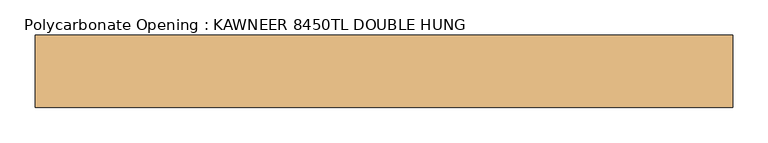
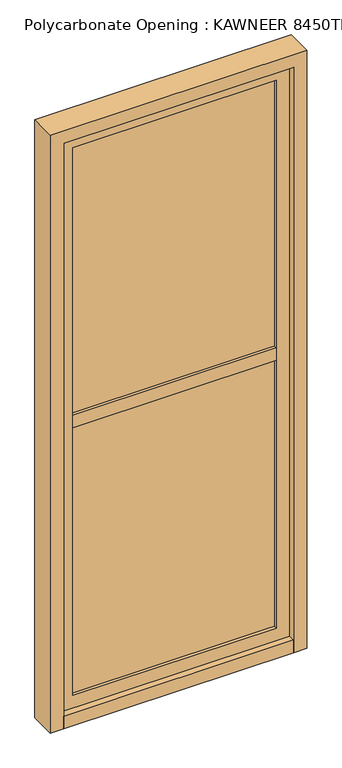
"""IFC4 building model written with IfcOpenShell, lengths in millimetres: door geometry, Polycarbonate Opening : KAWNEER 8450TL DOUBLE HUNG."""

from ifc_helpers import new_model, si_unit, frame, origin, origin_with_axes, place, context, project, spatial, polyline, outline, extrude, source, transform, mapped, element, save


def polycarbonate_opening_kawneer_8450tl_double_hung_a71d8d07(model_context):
    return source(origin(), model_context, "Body", "SweptSolid", [
        extrude(outline(polyline([(440.1908884, 12.7), (440.1908884, -12.7), (-440.1908884, -12.7), (-440.1908884, 12.7), (440.1908884, 12.7)])), frame((0.0, 0.0, 50.8), z_axis=(0.0, 0.0, 1.0), x_axis=(1.0, 0.0, 0.0)), (0.0, 0.0, 1.0), 2318.3403955),
        extrude(outline(polyline([(2369.1403955, -440.1908884), (0.0, -440.1908884), (0.0, 440.1908884), (2369.1403955, 440.1908884), (2369.1403955, -440.1908884)]), holes=[polyline([(101.6, 389.3908884), (101.6, -389.3908884), (2318.3403955, -389.3908884), (2318.3403955, 389.3908884), (101.6, 389.3908884)])]), frame((0.0, -25.4, 0.0), z_axis=(0.0, 1.0, 0.0), x_axis=(0.0, 0.0, 1.0)), (0.0, 0.0, 1.0), 50.8),
        extrude(outline(polyline([(2419.9403955, 490.9908884), (2419.9403955, -490.9908884), (0.0, -490.9908884), (0.0, -440.1908884), (2369.1403955, -440.1908884), (2369.1403955, 440.1908884), (0.0, 440.1908884), (0.0, 490.9908884), (2419.9403955, 490.9908884)])), frame((0.0, -50.8, 0.0), z_axis=(0.0, 1.0, 0.0), x_axis=(0.0, 0.0, 1.0)), (0.0, 0.0, 1.0), 101.6),
        extrude(outline(polyline([(440.1908884, 50.8), (440.1908884, -50.8), (-440.1908884, -50.8), (-440.1908884, 50.8), (440.1908884, 50.8)])), origin_with_axes(), (0.0, 0.0, 1.0), 50.8),
        extrude(outline(polyline([(389.3908884, 25.4), (389.3908884, -25.4), (-389.3908884, -25.4), (-389.3908884, 25.4), (389.3908884, 25.4)])), frame((0.0, 0.0, 1184.5701977), z_axis=(0.0, 0.0, 1.0), x_axis=(1.0, 0.0, 0.0)), (0.0, 0.0, 1.0), 50.8),
    ])


if __name__ == "__main__":
    model = new_model("IFC4")
    model_context = context("Model", 3, world=origin())
    ifc_project = project(units=[si_unit("LENGTHUNIT", "METRE", prefix="MILLI")], contexts=[model_context])
    site = spatial("IfcSite", under=ifc_project)
    building = spatial("IfcBuilding", under=site)
    placement = place(None, origin())
    polycarbonate_opening_kawneer_8450tl_double_hung_shape = polycarbonate_opening_kawneer_8450tl_double_hung_a71d8d07(model_context)
    element("IfcDoor", 1, ObjectType="Polycarbonate Opening : KAWNEER 8450TL DOUBLE HUNG", at=placement, inside=building, context=model_context, shape_type="MappedRepresentation", body=[
        mapped(polycarbonate_opening_kawneer_8450tl_double_hung_shape, transform((0.0, 0.0, 0.0), x_axis=(1.0, 0.0, 0.0), y_axis=(0.0, 1.0, 0.0), z_axis=(0.0, 0.0, 1.0))),
    ])
    save(model, "model.ifc")

# Revit data of these elements
# Type "Polycarbonate Opening : KAWNEER 8450TL DOUBLE HUNG"
#   Type Mark = "59"
#   OD_DS_Door_Material = "ALUM./GLAZING"
#   OD_DS_Door_Type = "STOREFRONT - DOUBLE HUNG WINDOW"
#   OD_DS_Lockset = "POLE OPERATOR HARDWARE FOR TOP SASH; BOTTOM SASH MECHANICALLY FIXED"
#   Analytic Construction = "<None>"
#   offset [instance default] = 0' - 2"
#   Stile = 0' - 2"
#   Mullion Width = 0' - 2"
#   Mullion Depth = 0' - 4"
#   Opening Size [instance default] = 5' - 1.50212"
#   Door Width [instance default] = 5' - 1.50212"
#   Window ON/OFF = no
#   Door On/Off = yes
#   Mullion Material = DOUBLE HUNG (CLEAR ANODIZED ALUM) - TEMPERED INSULATED GLAZING (CARDINAL GLASS LoĒ²-240\nOR EQUIVALENT)
#   Glass Material = TEMPERED INSULATED GLAZING (CARDINAL GLASS LoĒ²-240\nOR EQUIVALENT)
#   Door Material = DOUBLE HUNG (CLEAR ANODIZED ALUM) - TEMPERED INSULATED GLAZING (CARDINAL GLASS LoĒ²-240\nOR EQUIVALENT)
# Element 1 (IfcDoor, "Polycarbonate Opening : KAWNEER 8450TL DOUBLE HUNG")
#   offset = 0' - 0"
#   Materials on its faces: "DOUBLE HUNG (CLEAR ANODIZED ALUM) - TEMPERED INSULATED GLAZING (CARDINAL GLASS LoĒ²-240\nOR EQUIVALENT)", "TEMPERED INSULATED GLAZING (CARDINAL GLASS LoĒ²-240\nOR EQUIVALENT)"
# Materials
#   "DOUBLE HUNG (CLEAR ANODIZED ALUM) - TEMPERED INSULATED GLAZING (CARDINAL GLASS LoĒ²-240\nOR EQUIVALENT)": class "Metal", colour RGB 244 244 244, transparency 0, Description = "Aluminum 6061", Cost = 0
#   "TEMPERED INSULATED GLAZING (CARDINAL GLASS LoĒ²-240\nOR EQUIVALENT)": class "Glass", colour RGB 196 205 210, transparency 0.85, Description = "Soda Lime Glass", Cost = 0
